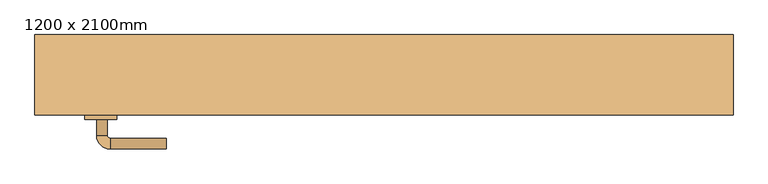
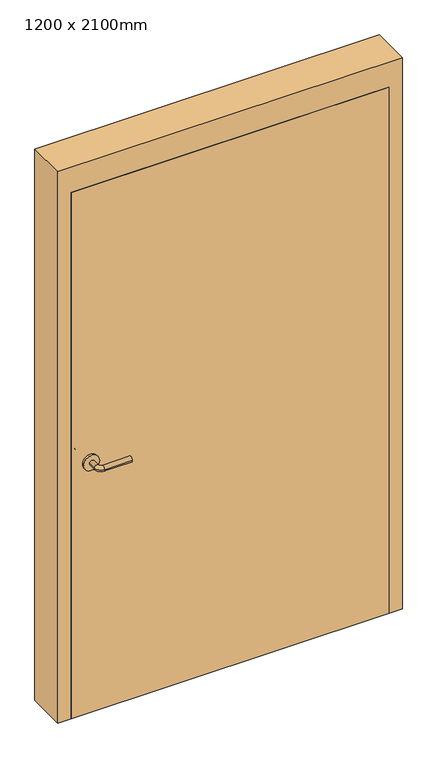
"""IFC4 building model written with IfcOpenShell, lengths in millimetres: door geometry, M_Puerta-De_paso-Simple-Paneles_planos : 1200 x 2100mm."""

from ifc_helpers import new_model, si_unit, point, frame, frame_2d, origin, origin_with_axes, place, context, project, spatial, polyline, circle_curve, ellipse_curve, trimmed, segment, composite_curve, outline, extrude, faceted_brep, source, transform, mapped, element, save
from ifc_brep_helpers import plane_surface, cylinder_surface, revolved_surface, advanced_brep


def door_1200_x_2100mm_64a0398e(model_context):
    return source(origin(), model_context, "Body", "SolidModel", [
        advanced_brep(
        [(-534.990625, -3.35, 1000.0), (-514.990625, -3.35, 1000.0), (-534.990625, 26.65, 1000.0), (-514.990625, 26.65, 1000.0), (-509.990625, 31.65, 1000.0), (-509.990625, 51.65, 1000.0), (-404.990625, 51.65, 1000.0), (-404.990625, 31.65, 1000.0)],
        [
            (0, 1, circle_curve(frame((-524.990625, -3.35, 1000.0), z_axis=(0.0, -1.0, 0.0), x_axis=(1.0, 0.0, 0.0)), 10.0)),
            (1, 0, circle_curve(frame((-524.990625, -3.35, 1000.0), z_axis=(0.0, -1.0, 0.0), x_axis=(1.0, 0.0, 0.0)), 10.0)),
            (0, 2),
            (2, 3, circle_curve(frame((-524.990625, 26.65, 1000.0), z_axis=(0.0, -1.0, 0.0), x_axis=(1.0, 0.0, 0.0)), 10.0)),
            (3, 1),
            (3, 2, circle_curve(frame((-524.990625, 26.65, 1000.0), z_axis=(0.0, -1.0, 0.0), x_axis=(1.0, 0.0, 0.0)), 10.0)),
            (4, 3, circle_curve(frame((-509.990625, 26.65, 1000.0), z_axis=(0.0, 0.0, 1.0), x_axis=(-1.0, 0.0, 0.0)), 5.0)),
            (2, 5, circle_curve(frame((-509.990625, 26.65, 1000.0), z_axis=(0.0, 0.0, -1.0), x_axis=(-1.0, 0.0, 0.0)), 25.0)),
            (5, 4, circle_curve(frame((-509.990625, 41.65, 1000.0), z_axis=(-1.0, 0.0, 0.0), x_axis=(0.0, -1.0, 0.0)), 10.0)),
            (4, 5, circle_curve(frame((-509.990625, 41.65, 1000.0), z_axis=(-1.0, 0.0, 0.0), x_axis=(0.0, -1.0, 0.0)), 10.0)),
            (6, 7, circle_curve(frame((-404.990625, 41.65, 1000.0), z_axis=(1.0, 0.0, 0.0), x_axis=(0.0, -1.0, 0.0)), 10.0)),
            (7, 6, circle_curve(frame((-404.990625, 41.65, 1000.0), z_axis=(1.0, 0.0, 0.0), x_axis=(0.0, -1.0, 0.0)), 10.0)),
            (5, 6),
            (7, 4),
        ],
        [
            plane_surface(frame((-524.990625, -3.35, 1000.0), z_axis=(0.0, -1.0, 0.0), x_axis=(0.0, 0.0, 1.0))),
            cylinder_surface(frame((-524.990625, -3.35, 1000.0), z_axis=(0.0, -1.0, 0.0), x_axis=(1.0, 0.0, 0.0)), 10.0),
            revolved_surface(trimmed(ellipse_curve(frame((-524.990625, 26.65, 1000.0), z_axis=(0.0, -1.0, 0.0), x_axis=(1.0, 0.0, 0.0)), 10.0, 10.0), [point((-534.990625, 26.65, 1000.0))], [point((-514.990625, 26.65, 1000.0))], True, "CARTESIAN"), (-509.990625, 26.65, 1000.0), (0.0, 0.0, -1.0)),
            revolved_surface(trimmed(ellipse_curve(frame((-524.990625, 26.65, 1000.0), z_axis=(0.0, -1.0, 0.0), x_axis=(1.0, 0.0, 0.0)), 10.0, 10.0), [point((-514.990625, 26.65, 1000.0))], [point((-534.990625, 26.65, 1000.0))], True, "CARTESIAN"), (-509.990625, 26.65, 1000.0), (0.0, 0.0, -1.0)),
            plane_surface(frame((-404.990625, 41.65, 1000.0), z_axis=(1.0, 0.0, 0.0), x_axis=(0.0, 0.0, 1.0))),
            cylinder_surface(frame((-509.990625, 41.65, 1000.0), z_axis=(-1.0, 0.0, 0.0), x_axis=(0.0, -1.0, 0.0)), 10.0),
        ],
        [
            (0, [[1, 2]]),
            (1, [[-1, 3, 4, 5]]),
            (1, [[-2, -5, 6, -3]]),
            (2, [[7, -4, 8, 9]]),
            (3, [[-8, -6, -7, 10]]),
            (4, [[11, 12]]),
            (5, [[-9, 13, -12, 14]]),
            (5, [[-10, -14, -11, -13]]),
        ],
    ),
        extrude(outline(composite_curve([segment(trimmed(circle_curve(frame_2d((1000.0, -527.490625)), 30.0), [point((1000.0, -557.490625))], [point((1000.0, -497.490625))], False, "CARTESIAN"), True, "CONTINUOUS"), segment(trimmed(circle_curve(frame_2d((1000.0, -527.490625)), 30.0), [point((1000.0, -497.490625))], [point((1000.0, -557.490625))], False, "CARTESIAN"), True, "CONTINUOUS")], self_intersect=False)), frame((0.0, -11.35, 0.0), z_axis=(0.0, 1.0, 0.0), x_axis=(0.0, 0.0, 1.0)), (0.0, 0.0, 1.0), 8.0),
        advanced_brep(
        [(-534.990625, -64.35, 1000.0), (-514.990625, -64.35, 1000.0), (-514.990625, -94.35, 1000.0), (-534.990625, -94.35, 1000.0), (-509.990625, -99.35, 1000.0), (-509.990625, -119.35, 1000.0), (-404.990625, -119.35, 1000.0), (-404.990625, -99.35, 1000.0)],
        [
            (0, 1, circle_curve(frame((-524.990625, -64.35, 1000.0), z_axis=(0.0, 1.0, 0.0), x_axis=(1.0, 0.0, 0.0)), 10.0)),
            (1, 0, circle_curve(frame((-524.990625, -64.35, 1000.0), z_axis=(0.0, 1.0, 0.0), x_axis=(1.0, 0.0, 0.0)), 10.0)),
            (1, 2),
            (2, 3, circle_curve(frame((-524.990625, -94.35, 1000.0), z_axis=(0.0, 1.0, 0.0), x_axis=(1.0, 0.0, 0.0)), 10.0)),
            (3, 0),
            (3, 2, circle_curve(frame((-524.990625, -94.35, 1000.0), z_axis=(0.0, 1.0, 0.0), x_axis=(1.0, 0.0, 0.0)), 10.0)),
            (4, 5, circle_curve(frame((-509.990625, -109.35, 1000.0), z_axis=(-1.0, 0.0, 0.0), x_axis=(0.0, 1.0, 0.0)), 10.0)),
            (5, 3, circle_curve(frame((-509.990625, -94.35, 1000.0), z_axis=(0.0, 0.0, -1.0), x_axis=(-1.0, 0.0, 0.0)), 25.0)),
            (2, 4, circle_curve(frame((-509.990625, -94.35, 1000.0), z_axis=(0.0, 0.0, 1.0), x_axis=(-1.0, 0.0, 0.0)), 5.0)),
            (5, 4, circle_curve(frame((-509.990625, -109.35, 1000.0), z_axis=(-1.0, 0.0, 0.0), x_axis=(0.0, 1.0, 0.0)), 10.0)),
            (6, 7, circle_curve(frame((-404.990625, -109.35, 1000.0), z_axis=(1.0, 0.0, 0.0), x_axis=(0.0, 1.0, 0.0)), 10.0)),
            (7, 6, circle_curve(frame((-404.990625, -109.35, 1000.0), z_axis=(1.0, 0.0, 0.0), x_axis=(0.0, 1.0, 0.0)), 10.0)),
            (4, 7),
            (6, 5),
        ],
        [
            plane_surface(frame((-524.990625, -64.35, 1000.0), z_axis=(0.0, 1.0, 0.0), x_axis=(0.0, 0.0, 1.0))),
            cylinder_surface(frame((-524.990625, -64.35, 1000.0), z_axis=(0.0, 1.0, 0.0), x_axis=(1.0, 0.0, 0.0)), 10.0),
            revolved_surface(trimmed(ellipse_curve(frame((-524.990625, -94.35, 1000.0), z_axis=(0.0, -1.0, 0.0), x_axis=(1.0, 0.0, 0.0)), 10.0, 10.0), [point((-534.990625, -94.35, 1000.0))], [point((-514.990625, -94.35, 1000.0))], True, "CARTESIAN"), (-509.990625, -94.35, 1000.0), (0.0, 0.0, -1.0)),
            revolved_surface(trimmed(ellipse_curve(frame((-524.990625, -94.35, 1000.0), z_axis=(0.0, -1.0, 0.0), x_axis=(1.0, 0.0, 0.0)), 10.0, 10.0), [point((-514.990625, -94.35, 1000.0))], [point((-534.990625, -94.35, 1000.0))], True, "CARTESIAN"), (-509.990625, -94.35, 1000.0), (0.0, 0.0, -1.0)),
            plane_surface(frame((-404.990625, -109.35, 1000.0), z_axis=(1.0, 0.0, 0.0), x_axis=(0.0, 0.0, 1.0))),
            cylinder_surface(frame((-509.990625, -109.35, 1000.0), z_axis=(-1.0, 0.0, 0.0), x_axis=(0.0, 1.0, 0.0)), 10.0),
        ],
        [
            (0, [[1, 2]]),
            (1, [[3, 4, 5, -2]]),
            (1, [[-5, 6, -3, -1]]),
            (2, [[7, 8, -4, 9]]),
            (3, [[10, -9, -6, -8]]),
            (4, [[11, 12]]),
            (5, [[13, -11, 14, -7]]),
            (5, [[-14, -12, -13, -10]]),
        ],
    ),
        extrude(outline(composite_curve([segment(trimmed(circle_curve(frame_2d((1000.0, -527.490625)), 30.0), [point((1000.0, -557.490625))], [point((1000.0, -497.490625))], False, "CARTESIAN"), True, "CONTINUOUS"), segment(trimmed(circle_curve(frame_2d((1000.0, -527.490625)), 30.0), [point((1000.0, -497.490625))], [point((1000.0, -557.490625))], False, "CARTESIAN"), True, "CONTINUOUS")], self_intersect=False)), frame((0.0, -64.35, 0.0), z_axis=(0.0, 1.0, 0.0), x_axis=(0.0, 0.0, 1.0)), (0.0, 0.0, 1.0), 8.0),
        extrude(outline(polyline([(600.0, -11.35), (600.0, -56.35), (-600.0, -56.35), (-600.0, -11.35), (600.0, -11.35)])), origin_with_axes(), (0.0, 0.0, 1.0), 2100.0),
        faceted_brep([(600.0, -6.5875, 0.0), (584.125, -6.5875, 0.0), (584.125, 44.4375, 0.0), (600.0, 44.4375, 0.0), (600.0, 93.65, 0.0), (650.0, 93.65, 0.0), (650.0, -56.35, 0.0), (600.0, -56.35, 0.0), (600.0, -56.35, 2100.0), (600.0, -6.5875, 2100.0), (650.0, -56.35, 2200.0), (-650.0, -56.35, 2200.0), (-650.0, -56.35, 0.0), (-600.0, -56.35, 0.0), (-600.0, -56.35, 2100.0), (650.0, 93.65, 2200.0), (600.0, 93.65, 2100.0), (-600.0, 93.65, 2100.0), (-600.0, 93.65, 0.0), (-650.0, 93.65, 0.0), (-650.0, 93.65, 2200.0), (600.0, 44.4375, 2100.0), (584.125, 44.4375, 2084.125), (-584.125, 44.4375, 2084.125), (-584.125, 44.4375, 0.0), (-600.0, 44.4375, 0.0), (-600.0, 44.4375, 2100.0), (584.125, -6.5875, 2084.125), (-600.0, -6.5875, 2100.0), (-600.0, -6.5875, 0.0), (-584.125, -6.5875, 0.0), (-584.125, -6.5875, 2084.125)], [[[0, 1, 2, 3, 4, 5, 6, 7]], [[7, 8, 9, 0]], [[6, 10, 11, 12, 13, 14, 8, 7]], [[5, 15, 10, 6]], [[4, 16, 17, 18, 19, 20, 15, 5]], [[3, 21, 16, 4]], [[2, 22, 23, 24, 25, 26, 21, 3]], [[1, 27, 22, 2]], [[0, 9, 28, 29, 30, 31, 27, 1]], [[8, 14, 28, 9]], [[16, 21, 26, 17]], [[22, 27, 31, 23]], [[12, 19, 18, 25, 24, 30, 29, 13]], [[13, 29, 28, 14]], [[11, 20, 19, 12]], [[17, 26, 25, 18]], [[23, 31, 30, 24]], [[15, 20, 11, 10]]]),
    ])


if __name__ == "__main__":
    model = new_model("IFC4")
    model_context = context("Model", 3, world=origin())
    ifc_project = project(units=[si_unit("LENGTHUNIT", "METRE", prefix="MILLI")], contexts=[model_context])
    site = spatial("IfcSite", under=ifc_project)
    building = spatial("IfcBuilding", under=site)
    placement = place(None, origin())
    door_1200_x_2100mm_shape = door_1200_x_2100mm_64a0398e(model_context)
    element("IfcDoor", 1, ObjectType="M_Puerta-De_paso-Simple-Paneles_planos : 1200 x 2100mm", at=placement, inside=building, context=model_context, shape_type="MappedRepresentation", body=[
        mapped(door_1200_x_2100mm_shape, transform((0.0, 0.0, 0.0), x_axis=(1.0, 0.0, 0.0), y_axis=(0.0, 1.0, 0.0), z_axis=(0.0, 0.0, 1.0))),
    ])
    save(model, "model.ifc")

# Revit data of these elements
# Type "M_Puerta-De_paso-Simple-Paneles_planos : 1200 x 2100mm"
#   Type Mark = "46"
#   Analytic Construction = "Madera"
#   Thickness = 0.045 m
#   Thermal Resistance (R) = 0.455703 (m²·K)/W
#   Ángulo de batiente [instance default] = 90.00°
#   Altura del pasador = 1.00 m
#   Rough Width [instance default] = 1.30 m
#   Rough Height [instance default] = 2.20 m
#   Altura de hueco MF [instance default] = 0.10 m
#   Anchura de hueco MF [instance default] = 0.10 m
#   Cálculo de la incrustación [instance default] = 0.105 m
#   Incrustación de albañilería [instance default] = 0.025 m
#   Height = 2.10 m
#   Width = 1.20 m
#   Heat Transfer Coefficient (U) = 2.19465 W/(m²·K)
#   Profundidad del marco del albañilería = 0.15 m
#   Marco del albañilería [instance default] = yes
#   Function = 1
#   Marco de muro seco [instance default] = no
#   Material de panel = Madera - Abedul
#   Material de estructura = Metal - Acabado de pintura - Gris
#   Material de tirador = Aluminio 1
#   Visual Light Transmittance = 0
#   Solar Heat Gain Coefficient = 0
#   Wall Closure = (empty or 0)
# Element 1 (IfcDoor, "M_Puerta-De_paso-Simple-Paneles_planos : 1200 x 2100mm")
#   Materials on its faces: "Aluminio 1", "Metal - Acabado de pintura - Gris", "Madera - Abedul"
# Materials
#   "Madera - Abedul": class "Madera", colour RGB 173 132 96, transparency 0, Cost = 0
#   "Metal - Acabado de pintura - Gris": class "Pintura", colour RGB 178 178 178, transparency 0, Cost = 0
#   "Aluminio 1": class "Metal", colour RGB 244 245 246, transparency 0, Description = "Aluminio 6061", Cost = 0
